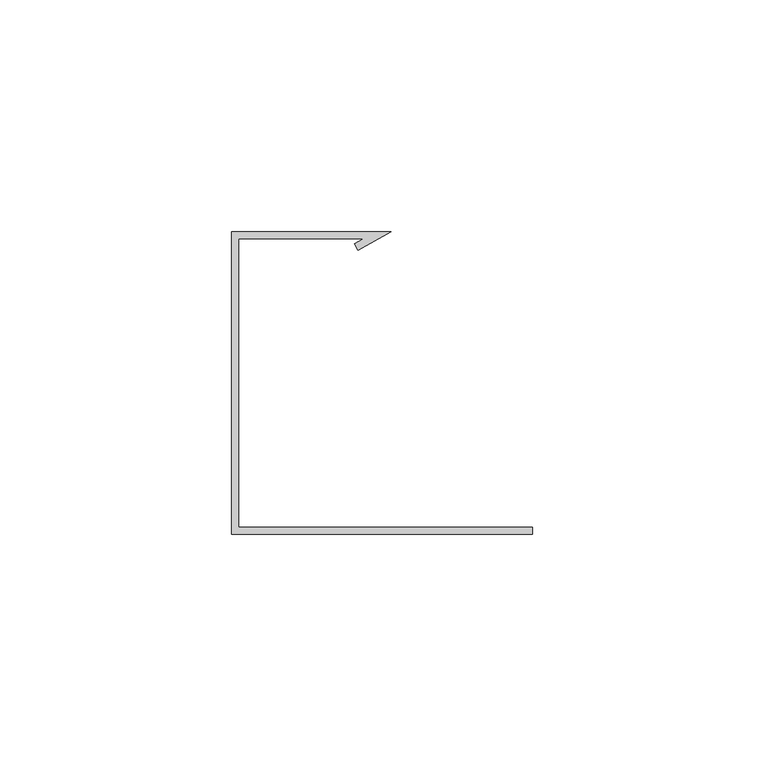
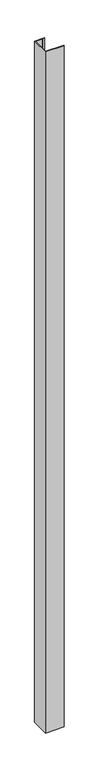
"""IFC4 building model written with IfcOpenShell, lengths in millimetres: proxy geometry, Generic Models 2:Generic Models 2:310765:Generic Models 2:310765 : Generic Models 2:Generic Models 2:310765:88 : Generic Models 2:Generic Models 2:310765:Generic Models 2:310765 : Generic Models 2:Generic Models 2:310765:300385."""

from ifc_helpers import new_model, si_unit, origin, origin_with_axes, place, context, project, spatial, polyline, outline, extrude, source, transform, mapped, element, save


def generic_models_9f78a53f(model_context):
    return source(origin(), model_context, "Body", "SweptSolid", [
        extrude(outline(polyline([(560295.811724, -530643.4262543), (560295.811724, -530577.9953608), (560330.2863675, -530577.9953608), (560323.2325076, -530582.0679087), (560322.4387576, -530580.6930934), (560324.3617369, -530579.5828608), (560297.399224, -530579.5828608), (560297.399224, -530641.8387543), (560360.899224, -530641.8387543), (560360.899224, -530643.4262543), (560295.811724, -530643.4262543)])), origin_with_axes(), (0.0, 0.0, 1.0), 2508.9309299),
    ])


if __name__ == "__main__":
    model = new_model("IFC4")
    model_context = context("Model", 3, world=origin())
    ifc_project = project(units=[si_unit("LENGTHUNIT", "METRE", prefix="MILLI")], contexts=[model_context])
    site = spatial("IfcSite", under=ifc_project)
    building = spatial("IfcBuilding", under=site)
    placement = place(None, origin())
    generic_models_shape = generic_models_9f78a53f(model_context)
    element("IfcBuildingElementProxy", 1, Name="Generic Models 2:Generic Models 2:310765:Generic Models 2:310765 : Generic Models 2:Generic Models 2:310765:88 : Generic Models 2:Generic Models 2:310765:Generic Models 2:310765 : Generic Models 2:Generic Models 2:310765:300385", ObjectType="Generic Models 2:Generic Models 2:310765:Generic Models 2:310765 : Generic Models 2:Generic Models 2:310765:88 : Generic Models 2:Generic Models 2:310765:Generic Models 2:310765 : Generic Models 2:Generic Models 2:310765:300385", at=placement, inside=building, context=model_context, shape_type="MappedRepresentation", body=[
        mapped(generic_models_shape, transform((0.0, 0.0, 0.0), x_axis=(1.0, 0.0, 0.0), y_axis=(0.0, 1.0, 0.0), z_axis=(0.0, 0.0, 1.0))),
    ])
    save(model, "model.ifc")

# Revit data of these elements
# Type "Generic Models 2:Generic Models 2:310765:Generic Models 2:310765 : Generic Models 2:Generic Models 2:310765:88 : Generic Models 2:Generic Models 2:310765:Generic Models 2:310765 : Generic Models 2:Generic Models 2:310765:300385"
#   NameOverride = "Generic Models 2:Generic Models 2:310765:Generic Models 2:310765 : Generic Models 2:Generic Models 2:310765:300385"
#   ObjectTypeOverride = "Generic Models 2:310765 : Generic Models 2:Generic Models 2:310765"
#   Reference = "Generic Models 2"
#   Tag = "300385"
# Element 1 (IfcBuildingElementProxy, "Generic Models 2:Generic Models 2:310765:Generic Models 2:310765 : Generic Models 2:Generic Models 2:310765:88 : Generic Models 2:Generic Models 2:310765:Generic Models 2:310765 : Generic Models 2:Generic Models 2:310765:300385")
#   Materials on its faces: "JAMB TRIM"
# Materials
#   "JAMB TRIM": class "Unassigned", colour RGB 210 209 208, transparency 0, Cost = 0
